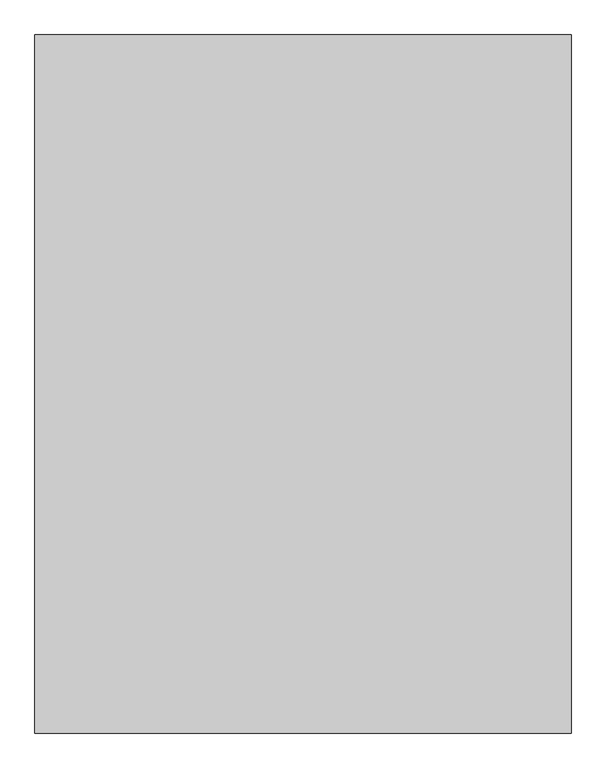
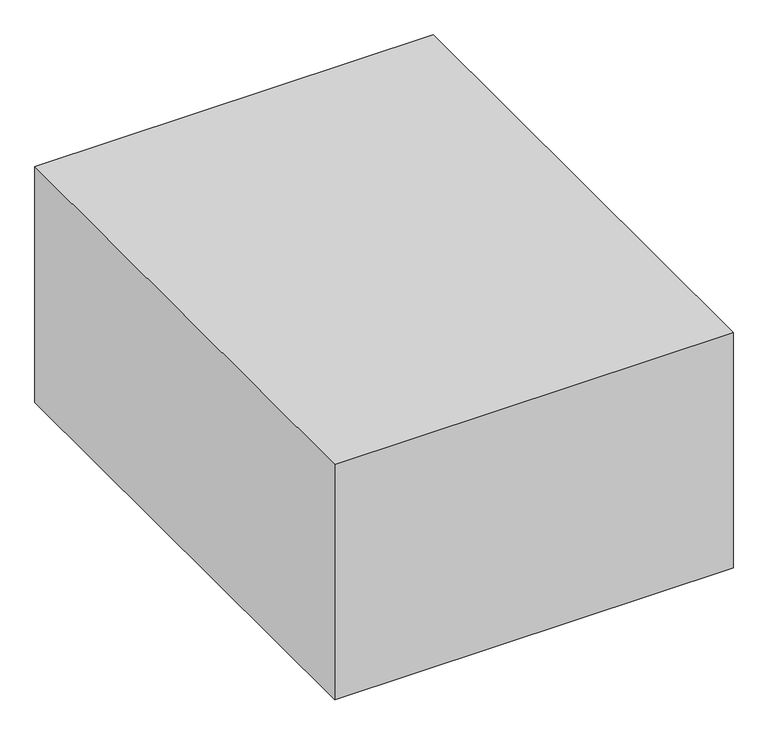
"""IFC4 building model written with IfcOpenShell, lengths in millimetres: proxy geometry, Space Planning Box_hec : Space Planning Box_hec."""

from ifc_helpers import new_model, si_unit, origin, origin_with_axes, place, context, project, spatial, polyline, outline, extrude, source, transform, mapped, element, save


def generic_models_72d488a7(model_context):
    return source(origin(), model_context, "Body", "SweptSolid", [
        extrude(outline(polyline([(4800.0, 6250.0), (4800.0, -6250.0), (-4800.0, -6250.0), (-4800.0, 6250.0), (4800.0, 6250.0)])), origin_with_axes(), (0.0, 0.0, 1.0), 6000.0),
    ])


if __name__ == "__main__":
    model = new_model("IFC4")
    model_context = context("Model", 3, world=origin())
    ifc_project = project(units=[si_unit("LENGTHUNIT", "METRE", prefix="MILLI")], contexts=[model_context])
    site = spatial("IfcSite", under=ifc_project)
    building = spatial("IfcBuilding", under=site)
    placement = place(None, origin())
    generic_models_shape = generic_models_72d488a7(model_context)
    element("IfcBuildingElementProxy", 1, Name="Space Planning Box_hec : Space Planning Box_hec", ObjectType="Space Planning Box_hec : Space Planning Box_hec", at=placement, inside=building, context=model_context, shape_type="MappedRepresentation", body=[
        mapped(generic_models_shape, transform((0.0, 0.0, 0.0), x_axis=(1.0, 0.0, 0.0), y_axis=(0.0, 1.0, 0.0), z_axis=(0.0, 0.0, 1.0))),
    ])
    save(model, "model.ifc")

# Revit data of these elements
# Type "Space Planning Box_hec : Space Planning Box_hec"
#   Type Comments = "..."
#   Room Name [instance default] = "?"
#   Interior Finish [instance default] = ""
#   Exterior Finish [instance default] = ""
#   Department [instance default] = ""
#   Assembly Code = "..."
#   Width [instance default] = 1524 mm
#   Program Area [instance default] = 0.00 m²
#   Length [instance default] = 1524 mm
#   Height [instance default] = 1524 mm
#   Area [instance default] = 2.32258 m²
#   Fill Color [instance default] = Cyan
#   Default Elevation = 0
# Element 1 (IfcBuildingElementProxy, "Space Planning Box_hec : Space Planning Box_hec")
#   Room Name = "Engineer Room"
#   Interior Finish = "IF3"
#   Exterior Finish = "EF1"
#   Department = "CI"
#   Width = 9600 mm
#   Program Area = 120.00 m²
#   Length = 12500 mm
#   Height = 6000 mm
#   Area = 120.00 m²
#   Fill Color = Lime
#   Materials on its faces: "Lime"
# Materials
#   "Cyan": class "Generic", colour RGB 0 255 255, transparency 0.2, Cost = 0
#   "Lime": class "Generic", colour RGB 0 255 0, transparency 0.2, Cost = 0
